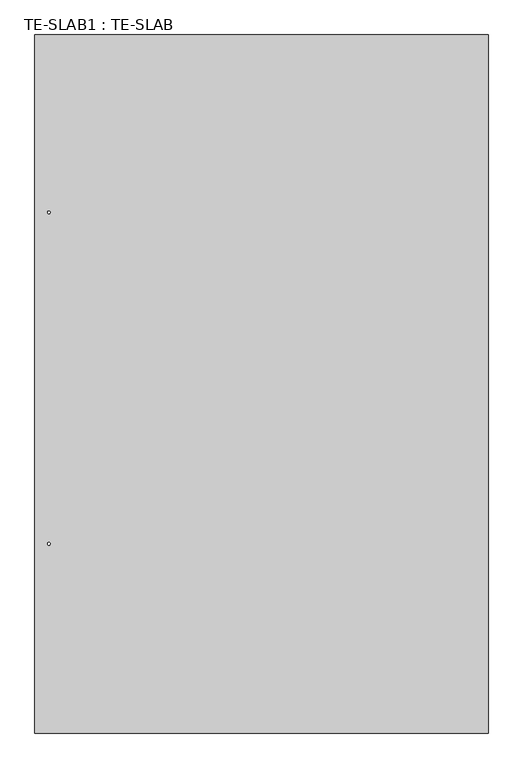
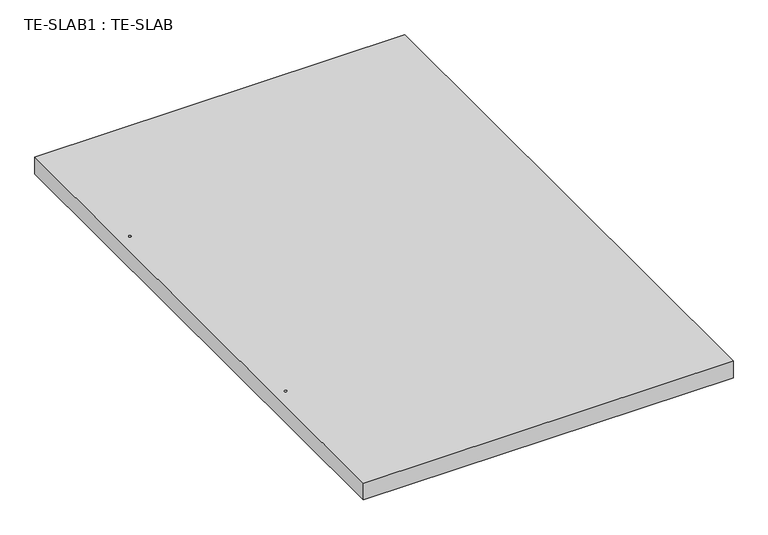
"""IFC4 building model written with IfcOpenShell, lengths in millimetres: proxy geometry, TE-SLAB1 : TE-SLAB."""

from ifc_helpers import new_model, si_unit, point, frame, frame_2d, origin, place, context, project, spatial, polyline, circle_curve, trimmed, segment, composite_curve, outline, extrude, source, transform, mapped, element, save


def te_slab1_te_slab_309ed248(model_context):
    return source(origin(), model_context, "Body", "SweptSolid", [
        extrude(outline(polyline([(590392.841184, -531594.7663841), (590392.841184, -536490.6163841), (587211.6785991, -536490.6163841), (587211.6785991, -531594.7663841), (590392.841184, -531594.7663841)]), holes=[composite_curve([segment(trimmed(circle_curve(frame_2d((587309.5435739, -532839.3663841)), 9.525), [point((587300.0185739, -532839.3663841))], [point((587319.0685739, -532839.3663841))], True, "CARTESIAN"), True, "CONTINUOUS"), segment(trimmed(circle_curve(frame_2d((587309.5435739, -532839.3663841)), 9.525), [point((587319.0685739, -532839.3663841))], [point((587300.0185739, -532839.3663841))], True, "CARTESIAN"), True, "CONTINUOUS")], self_intersect=False), composite_curve([segment(trimmed(circle_curve(frame_2d((587309.5435739, -535163.4663841)), 9.525), [point((587300.0185739, -535163.4663841))], [point((587319.0685739, -535163.4663841))], True, "CARTESIAN"), True, "CONTINUOUS"), segment(trimmed(circle_curve(frame_2d((587309.5435739, -535163.4663841)), 9.525), [point((587319.0685739, -535163.4663841))], [point((587300.0185739, -535163.4663841))], True, "CARTESIAN"), True, "CONTINUOUS")], self_intersect=False)]), frame((0.0, 0.0, -152.4), z_axis=(0.0, 0.0, 1.0), x_axis=(1.0, 0.0, 0.0)), (0.0, 0.0, 1.0), 152.4),
    ])


if __name__ == "__main__":
    model = new_model("IFC4")
    model_context = context("Model", 3, world=origin())
    ifc_project = project(units=[si_unit("LENGTHUNIT", "METRE", prefix="MILLI")], contexts=[model_context])
    site = spatial("IfcSite", under=ifc_project)
    building = spatial("IfcBuilding", under=site)
    placement = place(None, origin())
    te_slab1_te_slab_shape = te_slab1_te_slab_309ed248(model_context)
    element("IfcBuildingElementProxy", 1, Name="TE-SLAB1 : TE-SLAB", ObjectType="TE-SLAB1 : TE-SLAB", at=placement, inside=building, context=model_context, shape_type="MappedRepresentation", body=[
        mapped(te_slab1_te_slab_shape, transform((0.0, 0.0, 0.0), x_axis=(1.0, 0.0, 0.0), y_axis=(0.0, 1.0, 0.0), z_axis=(0.0, 0.0, 1.0))),
    ])
    save(model, "model.ifc")

# Revit data of these elements
# Element 1 (IfcBuildingElementProxy, "TE-SLAB1 : TE-SLAB")
#   Materials on its faces: "CONC, AIR-ENTRAINED_3500PSI #4@16\"EW"
# Materials
#   "CONC, AIR-ENTRAINED_3500PSI #4@16\"EW": class "Generic", colour RGB 145 145 143, transparency 0, Cost = 0
